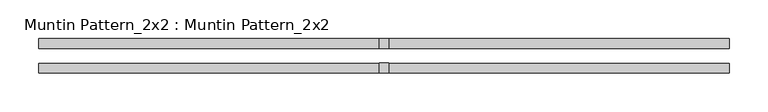
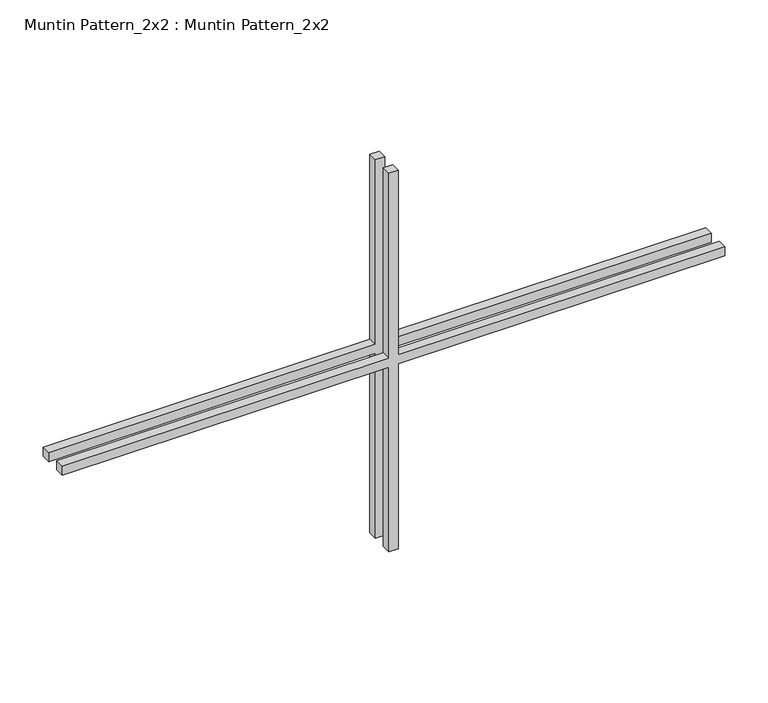
"""IFC4 building model written with IfcOpenShell, lengths in millimetres: proxy geometry, Muntin Pattern_2x2 : Muntin Pattern_2x2."""

import ifcopenshell
import ifcopenshell.guid

model = None  # the IFC model being written
_history = None  # IfcOwnerHistory: only IFC2X3 demands one
_inside = {}  # id of a spatial element -> (the spatial element, [elements in it])
_under = {}  # id of a project, library or spatial element -> (it, [spatial elements below it])
_declared = {}  # id of a project -> (the project, [libraries it declares])
_typed = {}  # id of a type object -> (the type object, [elements of that type])
_made_of = {}  # id of a material, layer set ... -> (it, [elements and type objects made of it])


def new_model(schema):
    """Start an empty IFC model of exactly this schema.

    Asked for "IFC4X3", IfcOpenShell would pick the latest addendum, in which some entities
    have other attributes; the version numbers below select the first issue.
    IFC2X3 requires an IfcOwnerHistory on every rooted entity: one is made here for all.
    """
    global model, _history
    if schema == "IFC4X3":
        model = ifcopenshell.file(schema_version=(4, 3, 0, 0))
    else:
        model = ifcopenshell.file(schema=schema)
    _inside.clear()
    _under.clear()
    _declared.clear()
    _typed.clear()
    _made_of.clear()
    _history = None
    if model.schema == "IFC2X3":
        org = make("IfcOrganization", Name="unknown")
        user = make(
            "IfcPersonAndOrganization",
            ThePerson=make("IfcPerson", FamilyName="unknown"),
            TheOrganization=org,
        )
        app = make(
            "IfcApplication",
            ApplicationDeveloper=org,
            Version="unknown",
            ApplicationFullName="unknown",
            ApplicationIdentifier="unknown",
        )
        _history = make(
            "IfcOwnerHistory",
            OwningUser=user,
            OwningApplication=app,
            ChangeAction="ADDED",
            CreationDate=0,
        )
    return model


def make(cls, **values):
    """One entity of the class cls with the attributes given. An attribute that is None is left unset."""
    return model.create_entity(
        cls, **{name: value for name, value in values.items() if value is not None}
    )


def rooted(cls, **values):
    """An entity with a GlobalId (a new one), such as an element, a storey or a relation."""
    return make(cls, GlobalId=ifcopenshell.guid.new(), OwnerHistory=_history, **values)


def si_unit(unit_type, name, prefix=None):
    """IfcSIUnit, for example si_unit("LENGTHUNIT", "METRE", prefix="MILLI")."""
    return make("IfcSIUnit", UnitType=unit_type, Prefix=prefix, Name=name)


def assignment(units):
    """IfcUnitAssignment: the units of a project."""
    return None if units is None else make("IfcUnitAssignment", Units=units)


def point(xyz):
    """IfcCartesianPoint."""
    return None if xyz is None else make("IfcCartesianPoint", Coordinates=xyz)


def direction(xyz):
    """IfcDirection."""
    return None if xyz is None else make("IfcDirection", DirectionRatios=xyz)


def frame(location, z_axis=None, x_axis=None):
    """IfcAxis2Placement3D, a coordinate frame: its origin and axes. An axis left out is left unset."""
    return make(
        "IfcAxis2Placement3D",
        Location=point(location),
        Axis=direction(z_axis),
        RefDirection=direction(x_axis),
    )


def origin():
    """The frame at (0, 0, 0) with its axes left unset."""
    return frame((0.0, 0.0, 0.0))


def place(relative_to, where):
    """IfcLocalPlacement: puts the frame where relative to a parent placement (None: the world)."""
    return make(
        "IfcLocalPlacement", PlacementRelTo=relative_to, RelativePlacement=where
    )


def context(
    kind, dimensions, precision=None, world=None, true_north=None, identifier=None
):
    """IfcGeometricRepresentationContext, for example the 3D "Model" context."""
    return make(
        "IfcGeometricRepresentationContext",
        ContextIdentifier=identifier,
        ContextType=kind,
        CoordinateSpaceDimension=dimensions,
        Precision=precision,
        WorldCoordinateSystem=world,
        TrueNorth=true_north,
    )


def project(units=None, contexts=None):
    """IfcProject with its units and contexts."""
    return rooted(
        "IfcProject",
        Name="project",
        RepresentationContexts=contexts,
        UnitsInContext=assignment(units),
    )


def spatial(cls, under=None, at=None, **own):
    """A site, building, storey or space (cls), placed at a placement, below another one or the project."""
    s = rooted(cls, ObjectPlacement=at, **own)
    if under is not None:
        _under.setdefault(under.id(), (under, []))[1].append(s)
    return s


def polyline(points):
    """IfcPolyline through the points."""
    return make("IfcPolyline", Points=[point(p) for p in points])


def outline(outer, holes=None, kind="AREA"):
    """IfcArbitraryClosedProfileDef: a profile drawn as a closed curve; with holes, ...WithVoids."""
    if holes is None:
        return make("IfcArbitraryClosedProfileDef", ProfileType=kind, OuterCurve=outer)
    return make(
        "IfcArbitraryProfileDefWithVoids",
        ProfileType=kind,
        OuterCurve=outer,
        InnerCurves=holes,
    )


def extrude(swept, where, along, depth):
    """IfcExtrudedAreaSolid: the profile swept, set in the frame where, extruded along a direction by depth."""
    return make(
        "IfcExtrudedAreaSolid",
        SweptArea=swept,
        Position=where,
        ExtrudedDirection=direction(along),
        Depth=depth,
    )


def shape(context_of_items, identifier, shape_type, items):
    """IfcShapeRepresentation: the items that make up one representation, for example the "Body"."""
    return make(
        "IfcShapeRepresentation",
        ContextOfItems=context_of_items,
        RepresentationIdentifier=identifier,
        RepresentationType=shape_type,
        Items=items,
    )


def source(mapping_origin, context_of_items, identifier, shape_type, items):
    """IfcRepresentationMap: a shape defined once, which mapped items show again and again."""
    return make(
        "IfcRepresentationMap",
        MappingOrigin=mapping_origin,
        MappedRepresentation=shape(context_of_items, identifier, shape_type, items),
    )


def transform(
    local_origin,
    x_axis=None,
    y_axis=None,
    z_axis=None,
    scale=None,
    scale2=None,
    scale3=None,
    uniform=True,
):
    """IfcCartesianTransformationOperator3D, or its non-uniform kind. x_axis, y_axis, z_axis: its Axis1, 2, 3."""
    if uniform:
        return make(
            "IfcCartesianTransformationOperator3D",
            Axis1=direction(x_axis),
            Axis2=direction(y_axis),
            LocalOrigin=point(local_origin),
            Scale=scale,
            Axis3=direction(z_axis),
        )
    return make(
        "IfcCartesianTransformationOperator3DnonUniform",
        Axis1=direction(x_axis),
        Axis2=direction(y_axis),
        LocalOrigin=point(local_origin),
        Scale=scale,
        Axis3=direction(z_axis),
        Scale2=scale2,
        Scale3=scale3,
    )


def mapped(mapping_source, mapping_target):
    """IfcMappedItem: shows the shape of a source again, moved by a transform."""
    return make(
        "IfcMappedItem", MappingSource=mapping_source, MappingTarget=mapping_target
    )


def made_of(thing, what):
    """Note that an element or type object is made of a material, layer set ...; save() writes the relation."""
    if what is not None:
        _made_of.setdefault(what.id(), (what, []))[1].append(thing)
    return thing


def element(
    cls,
    number,
    at=None,
    inside=None,
    cuts=None,
    type_object=None,
    material=None,
    context=None,
    identifier="Body",
    shape_type=None,
    held_by="IfcProductDefinitionShape",
    body=None,
    shapes=None,
    **own,
):
    """One element of the class cls, such as IfcWall. Its Tag is "e" and its number.

    at: its placement. inside: the storey or other place that contains it. cuts: it is an
    opening in that element (IfcRelVoidsElement). A single representation is given by context,
    identifier, shape_type and body (its items); several are given by shapes. held_by: the class
    of the entity that holds the representations. save() writes the other relations.
    """
    e = rooted(cls, Tag="e%d" % number, ObjectPlacement=at, **own)
    if body is not None:
        shapes = [shape(context, identifier, shape_type, body)]
    if shapes is not None:
        e.Representation = make(held_by, Representations=shapes)
    if inside is not None:
        _inside.setdefault(inside.id(), (inside, []))[1].append(e)
    if cuts is not None:
        rooted(
            "IfcRelVoidsElement", RelatingBuildingElement=cuts, RelatedOpeningElement=e
        )
    if type_object is not None:
        _typed.setdefault(type_object.id(), (type_object, []))[1].append(e)
    return made_of(e, material)


def aggregate(whole, parts):
    """IfcRelAggregates: a whole, such as a stair, and the parts it consists of."""
    return rooted("IfcRelAggregates", RelatingObject=whole, RelatedObjects=parts)


def save(model, path):
    """Write the relations noted so far, then the file.

    IfcRelAggregates (storeys below a building ...), IfcRelContainedInSpatialStructure (elements
    in a storey), IfcRelDefinesByType, IfcRelAssociatesMaterial and IfcRelDeclares: one each for
    every whole, place, type object, material and project.
    """
    for whole, parts in _under.values():
        aggregate(whole, parts)
    for where, things in _inside.values():
        rooted(
            "IfcRelContainedInSpatialStructure",
            RelatedElements=things,
            RelatingStructure=where,
        )
    for kind, things in _typed.values():
        rooted("IfcRelDefinesByType", RelatedObjects=things, RelatingType=kind)
    for what, things in _made_of.values():
        rooted("IfcRelAssociatesMaterial", RelatedObjects=things, RelatingMaterial=what)
    for by, libraries in _declared.values():
        rooted("IfcRelDeclares", RelatingContext=by, RelatedDefinitions=libraries)
    model.write(path)


def muntin_pattern_2x2_muntin_pattern_2x2_50d3873d(model_context):
    return source(origin(), model_context, "Body", "SweptSolid", [
        extrude(outline(polyline([(274.6375, -6.35), (274.6375, -444.5), (261.9375, -444.5), (261.9375, -6.35), (0.0, -6.35), (0.0, 6.35), (261.9375, 6.35), (261.9375, 444.5), (274.6375, 444.5), (274.6375, 6.35), (536.575, 6.35), (536.575, -6.35), (274.6375, -6.35)])), frame((0.0, -22.225, 0.0), z_axis=(0.0, 1.0, 0.0), x_axis=(0.0, 0.0, 1.0)), (0.0, 0.0, 1.0), 12.7),
        extrude(outline(polyline([(274.6375, -6.35), (274.6375, -444.5), (261.9375, -444.5), (261.9375, -6.35), (0.0, -6.35), (0.0, 6.35), (261.9375, 6.35), (261.9375, 444.5), (274.6375, 444.5), (274.6375, 6.35), (536.575, 6.35), (536.575, -6.35), (274.6375, -6.35)])), frame((0.0, 9.525, 0.0), z_axis=(0.0, 1.0, 0.0), x_axis=(0.0, 0.0, 1.0)), (0.0, 0.0, 1.0), 12.7),
    ])


if __name__ == "__main__":
    model = new_model("IFC4")
    model_context = context("Model", 3, world=origin())
    ifc_project = project(units=[si_unit("LENGTHUNIT", "METRE", prefix="MILLI")], contexts=[model_context])
    site = spatial("IfcSite", under=ifc_project)
    building = spatial("IfcBuilding", under=site)
    placement = place(None, origin())
    muntin_pattern_2x2_muntin_pattern_2x2_shape = muntin_pattern_2x2_muntin_pattern_2x2_50d3873d(model_context)
    element("IfcBuildingElementProxy", 1, Name="Muntin Pattern_2x2 : Muntin Pattern_2x2", ObjectType="Muntin Pattern_2x2 : Muntin Pattern_2x2", at=placement, inside=building, context=model_context, shape_type="MappedRepresentation", body=[
        mapped(muntin_pattern_2x2_muntin_pattern_2x2_shape, transform((0.0, 0.0, 0.0), x_axis=(1.0, 0.0, 0.0), y_axis=(0.0, 1.0, 0.0), z_axis=(0.0, 0.0, 1.0))),
    ])
    save(model, "model.ifc")

# Revit data of these elements
# Type "Muntin Pattern_2x2 : Muntin Pattern_2x2"
#   Width [instance default] = 4' - 0"
#   Thickness = 0' - 0 1/2"
#   Height [instance default] = 4' - 0"
#   Distance = 0' - 0 3/4"
#   Interior Material [instance default] = none
#   Exterior Material [instance default] = none
# Element 1 (IfcBuildingElementProxy, "Muntin Pattern_2x2 : Muntin Pattern_2x2")
#   Width = 2' - 11"
#   Height = 1' - 9 1/8"
#   Interior Material = Wood - Stained
#   Exterior Material = Clad - White
#   Materials on its faces: "Clad - White", "Wood - Stained"
# Materials
#   "Clad - White": class "Wood", colour RGB 242 242 238, transparency 0, Cost = 0
#   "Wood - Stained": class "Wood", colour RGB 224 178 126, transparency 0, Cost = 0
